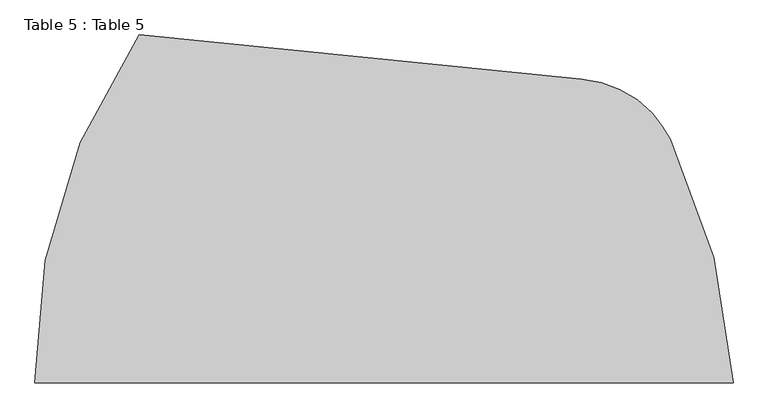
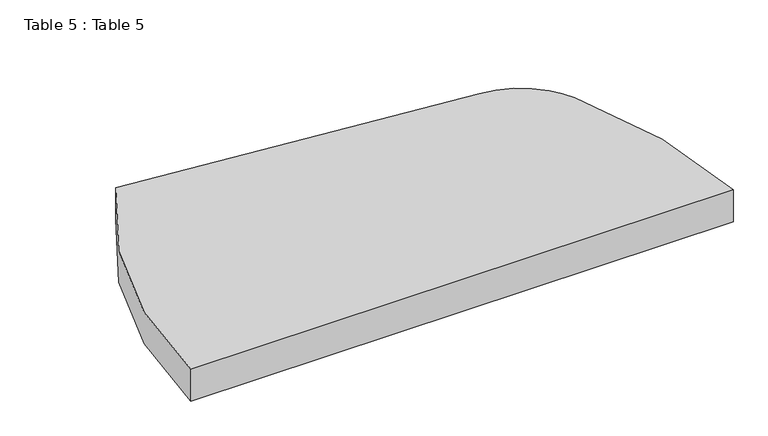
"""IFC4 building model written with IfcOpenShell, lengths in millimetres: furniture geometry, Table 5 : Table 5."""

from ifc_helpers import new_model, si_unit, point, frame, frame_2d, origin, place, context, project, spatial, polyline, circle_curve, trimmed, segment, composite_curve, outline, extrude, source, transform, mapped, element, save


def table_5_table_5_6309b113(model_context):
    return source(origin(), model_context, "Body", "SweptSolid", [
        extrude(outline(composite_curve([segment(trimmed(circle_curve(frame_2d((-566.0798185, -5842.2993677)), 250.0), [point((-548.1347224, -5592.9442524))], [point((-383.4886467, -5671.5350155))], False, "CARTESIAN"), True, "CONTINUOUS"), segment(trimmed(circle_curve(frame_2d((-566.0798185, -5842.2993677)), 250.0), [point((-383.4886467, -5671.5350155))], [point((-341.6614078, -5732.1341422))], False, "CARTESIAN"), True, "CONTINUOUS"), segment(trimmed(circle_curve(frame_2d((-1644.999673, -6371.9326037)), 1451.9065758), [point((-341.6614078, -5732.1341422))], [point((-194.8932516, -6299.6548647))], False, "CARTESIAN"), True, "CONTINUOUS"), segment(polyline([(-194.8932516, -6299.6548647), (-1819.3632624, -6299.6548647)]), True, "CONTINUOUS"), segment(trimmed(circle_curve(frame_2d((-433.9008548, -6272.7932629)), 1385.7227821), [point((-1819.3632624, -6299.6548647))], [point((-1576.9945112, -5489.4896683))], False, "CARTESIAN"), True, "CONTINUOUS"), segment(trimmed(circle_curve(frame_2d((760.0219024, 12584.475549)), 18224.4304271), [point((-1576.9945112, -5489.4896683))], [point((-548.1347224, -5592.9442524))], True, "CARTESIAN"), True, "CONTINUOUS")], self_intersect=False)), frame((0.0, 0.0, 500.0), z_axis=(0.0, 0.0, 1.0), x_axis=(1.0, 0.0, 0.0)), (0.0, 0.0, 1.0), 100.0),
    ])


if __name__ == "__main__":
    model = new_model("IFC4")
    model_context = context("Model", 3, world=origin())
    ifc_project = project(units=[si_unit("LENGTHUNIT", "METRE", prefix="MILLI")], contexts=[model_context])
    site = spatial("IfcSite", under=ifc_project)
    building = spatial("IfcBuilding", under=site)
    placement = place(None, origin())
    table_5_table_5_shape = table_5_table_5_6309b113(model_context)
    element("IfcFurniture", 1, ObjectType="Table 5 : Table 5", at=placement, inside=building, context=model_context, shape_type="MappedRepresentation", body=[
        mapped(table_5_table_5_shape, transform((0.0, 0.0, 0.0), x_axis=(1.0, 0.0, 0.0), y_axis=(0.0, 1.0, 0.0), z_axis=(0.0, 0.0, 1.0))),
    ])
    save(model, "model.ifc")

# Revit data of these elements
# Type "Table 5 : Table 5"
#   COBie.Type.CreatedBy = "design@eagle.com"
#   COBie.Type.CreatedOn = "2016-09-13T05:47:35"
#   COBie.Type.Name = "Furniture_Table 5_Table 5"
#   COBie.Type.Category = "23-40 70 14 64 11 : Office Furniture"
#   COBie.Type.Description = ""
#   COBie.Type.Manufacturer = ""
#   COBie.Type.ModelNumber = ""
#   COBie.Type.ReplacementCost = 0
#   COBie.Type = yes
